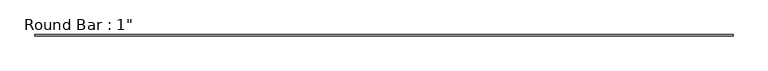
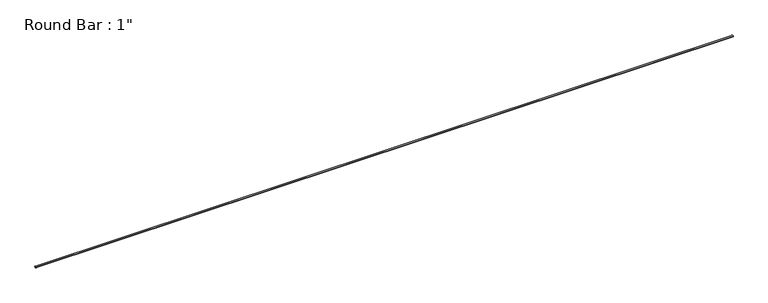
"""IFC4 building model written with IfcOpenShell, lengths in millimetres: member geometry."""

from ifc_helpers import new_model, si_unit, point, frame, origin, origin_2d, place, context, project, spatial, circle_curve, trimmed, segment, composite_curve, outline, extrude, source, transform, mapped, element, save


def member_a1e25d91(model_context):
    return source(origin(), model_context, "Body", "SweptSolid", [
        extrude(outline(composite_curve([segment(trimmed(circle_curve(origin_2d(), 12.7), [point((-12.7, 0.0))], [point((12.7, 0.0))], False, "CARTESIAN"), True, "CONTINUOUS"), segment(trimmed(circle_curve(origin_2d(), 12.7), [point((12.7, 0.0))], [point((-12.7, 0.0))], False, "CARTESIAN"), True, "CONTINUOUS")], self_intersect=False)), frame((-6152.7715595, 0.0, 0.0), z_axis=(1.0, 0.0, 0.0), x_axis=(0.0, 1.0, 0.0)), (0.0, 0.0, 1.0), 12305.543119),
    ])


if __name__ == "__main__":
    model = new_model("IFC4")
    model_context = context("Model", 3, world=origin())
    ifc_project = project(units=[si_unit("LENGTHUNIT", "METRE", prefix="MILLI")], contexts=[model_context])
    site = spatial("IfcSite", under=ifc_project)
    building = spatial("IfcBuilding", under=site)
    placement = place(None, origin())
    member_shape = member_a1e25d91(model_context)
    element("IfcMember", 1, ObjectType="Round Bar : 1\"", at=placement, inside=building, context=model_context, shape_type="MappedRepresentation", body=[
        mapped(member_shape, transform((0.0, 0.0, 0.0), x_axis=(1.0, 0.0, 0.0), y_axis=(0.0, 1.0, 0.0), z_axis=(0.0, 0.0, 1.0))),
    ])
    save(model, "model.ifc")

# Revit data of these elements
# Type "Round Bar : 1\""
#   Assembly Code = "B10"
#   W = 0
#   Start Extension Calculation [instance default] = 10' - 0"
#   Start Extension [instance default] = -0' - 0 1/2"
#   End Extension Calculation [instance default] = 10' - 0"
#   End Extension [instance default] = -0' - 0 1/2"
#   Length [instance default] = 5' - 0"
#   d = 0' - 1"
#   A = 0 SF
#   Structural Material [instance default] = Metal - Steel - ASTM A36
# Element 1 (IfcMember, "Round Bar : 1\"")
#   Materials on its faces: "Metal - Steel - ASTM A36"
# Materials
#   "Metal - Steel - ASTM A36": class "Metal", colour RGB 199 199 199, transparency 0
